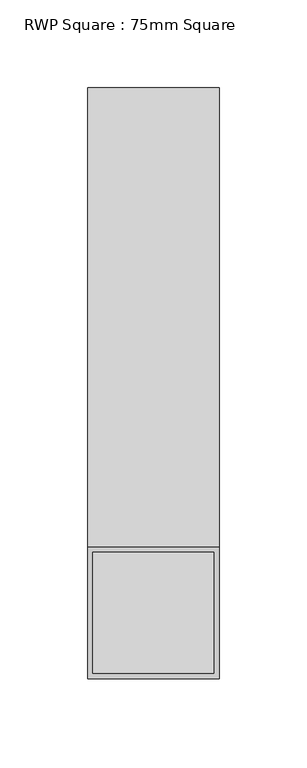
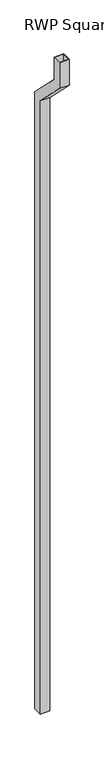
"""IFC4 building model written with IfcOpenShell, lengths in millimetres: proxy geometry, RWP Square : 75mm Square."""

from ifc_helpers import new_model, si_unit, origin, place, context, project, spatial, faceted_brep, source, transform, mapped, element, save


def rwp_square_75mm_square_53b424de(model_context):
    return source(origin(), model_context, "Body", "Brep", [
        faceted_brep([(37.5, -0.5, 0.0), (37.5, -75.5, 0.0), (-37.5, -75.5, 0.0), (-37.5, -0.5, 0.0), (34.5, -3.5, 0.0), (-34.5, -3.5, 0.0), (-34.5, -72.5, 0.0), (34.5, -72.5, 0.0), (-37.5, -0.5, 5153.5330086), (37.5, -0.5, 5153.5330086), (-37.5, -75.5, 5122.4669914), (-37.5, -337.5, 5384.4669914), (-37.5, -337.5, 5600.0), (-37.5, -262.5, 5600.0), (-37.5, -262.5, 5415.5330086), (37.5, -75.5, 5122.4669914), (37.5, -262.5, 5415.5330086), (37.5, -262.5, 5600.0), (37.5, -337.5, 5600.0), (37.5, -337.5, 5384.4669914), (34.5, -72.5, 5123.7096321), (34.5, -334.5, 5385.7096321), (34.5, -334.5, 5600.0), (34.5, -265.5, 5600.0), (34.5, -265.5, 5414.2903679), (34.5, -3.5, 5152.2903679), (-34.5, -72.5, 5123.7096321), (-34.5, -3.5, 5152.2903679), (-34.5, -265.5, 5414.2903679), (-34.5, -265.5, 5600.0), (-34.5, -334.5, 5600.0), (-34.5, -334.5, 5385.7096321)], [[[0, 1, 2, 3], [4, 5, 6, 7]], [[3, 8, 9, 0]], [[2, 10, 11, 12, 13, 14, 8, 3]], [[1, 15, 10, 2]], [[0, 9, 16, 17, 18, 19, 15, 1]], [[7, 20, 21, 22, 23, 24, 25, 4]], [[6, 26, 20, 7]], [[5, 27, 28, 29, 30, 31, 26, 6]], [[4, 25, 27, 5]], [[8, 14, 16, 9]], [[15, 19, 11, 10]], [[26, 31, 21, 20]], [[25, 24, 28, 27]], [[17, 13, 12, 18], [23, 22, 30, 29]], [[14, 13, 17, 16]], [[19, 18, 12, 11]], [[31, 30, 22, 21]], [[24, 23, 29, 28]]]),
    ])


if __name__ == "__main__":
    model = new_model("IFC4")
    model_context = context("Model", 3, world=origin())
    ifc_project = project(units=[si_unit("LENGTHUNIT", "METRE", prefix="MILLI")], contexts=[model_context])
    site = spatial("IfcSite", under=ifc_project)
    building = spatial("IfcBuilding", under=site)
    placement = place(None, origin())
    rwp_square_75mm_square_shape = rwp_square_75mm_square_53b424de(model_context)
    element("IfcBuildingElementProxy", 1, Name="RWP Square : 75mm Square", ObjectType="RWP Square : 75mm Square", at=placement, inside=building, context=model_context, shape_type="MappedRepresentation", body=[
        mapped(rwp_square_75mm_square_shape, transform((0.0, 0.0, 0.0), x_axis=(1.0, 0.0, 0.0), y_axis=(0.0, 1.0, 0.0), z_axis=(0.0, 0.0, 1.0))),
    ])
    save(model, "model.ifc")

# Revit data of these elements
# Type "RWP Square : 75mm Square"
#   Keynote = "R"
#   RWP Width = 75 mm
#   RWP Wall Thickness = 3 mm
#   RWP Depth = 75 mm
#   Offset Top = 300 mm
#   Offset Base = 38 mm
#   Height of RWP [instance default] = 5000 mm
#   Head Splayed Depth = 262 mm
#   Head Depth = 200 mm
#   Material RWP = Plastic - White
# Element 1 (IfcBuildingElementProxy, "RWP Square : 75mm Square")
#   Height of RWP = 5600 mm
#   Materials on its faces: "Plastic - White"
# Materials
#   "Plastic - White": class "Plastic", colour RGB 249 249 249, transparency 0
